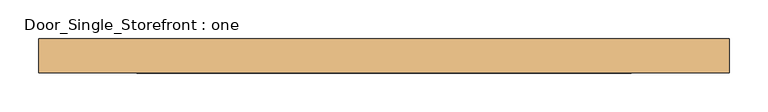
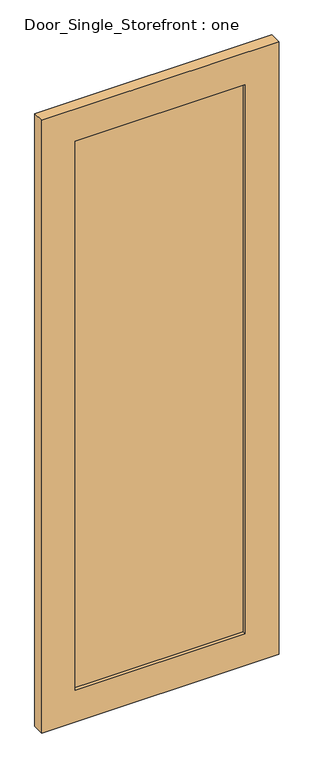
"""IFC4 building model written with IfcOpenShell, lengths in millimetres: door geometry, Door_Single_Storefront : one."""

from ifc_helpers import new_model, si_unit, frame, origin, place, context, project, spatial, polyline, outline, extrude, source, transform, mapped, element, save


def door_single_storefront_one_e372f670(model_context):
    return source(origin(), model_context, "Body", "SweptSolid", [
        extrude(outline(polyline([(319.88125, -6.35), (-319.88125, -6.35), (-319.88125, 12.7), (319.88125, 12.7), (319.88125, -6.35)])), frame((0.0, 0.0, 127.0), z_axis=(0.0, 0.0, 1.0), x_axis=(1.0, 0.0, 0.0)), (0.0, 0.0, 1.0), 2184.4),
        extrude(outline(polyline([(2438.4, -446.88125), (0.0, -446.88125), (0.0, 446.88125), (2438.4, 446.88125), (2438.4, -446.88125)]), holes=[polyline([(127.0, 319.88125), (127.0, -319.88125), (2311.4, -319.88125), (2311.4, 319.88125), (127.0, 319.88125)])]), frame((0.0, -19.05, 0.0), z_axis=(0.0, 1.0, 0.0), x_axis=(0.0, 0.0, 1.0)), (0.0, 0.0, 1.0), 44.45),
    ])


if __name__ == "__main__":
    model = new_model("IFC4")
    model_context = context("Model", 3, world=origin())
    ifc_project = project(units=[si_unit("LENGTHUNIT", "METRE", prefix="MILLI")], contexts=[model_context])
    site = spatial("IfcSite", under=ifc_project)
    building = spatial("IfcBuilding", under=site)
    placement = place(None, origin())
    door_single_storefront_one_shape = door_single_storefront_one_e372f670(model_context)
    element("IfcDoor", 1, ObjectType="Door_Single_Storefront : one", at=placement, inside=building, context=model_context, shape_type="MappedRepresentation", body=[
        mapped(door_single_storefront_one_shape, transform((0.0, 0.0, 0.0), x_axis=(1.0, 0.0, 0.0), y_axis=(0.0, 1.0, 0.0), z_axis=(0.0, 0.0, 1.0))),
    ])
    save(model, "model.ifc")

# Revit data of these elements
# Type "Door_Single_Storefront : one"
#   Type Mark = "27"
#   Analytic Construction = "<None>"
#   Stile_Width = 0' - 5"
#   Door_Thickness = 0' - 1 3/4"
#   Door_Offset = 0' - 1"
#   Glass_Material = SAFETY GLAZING
#   Frame_Material = INTERIOR GRADE ALUMINUM STOREFRONT W/ SAFETY GLAZING
#   Function = (empty or 0)
# Element 1 (IfcDoor, "Door_Single_Storefront : one")
#   Materials on its faces: "INTERIOR GRADE ALUMINUM STOREFRONT W/ SAFETY GLAZING", "SAFETY GLAZING"
# Materials
#   "SAFETY GLAZING": class "Glass", colour RGB 142 168 196, transparency 0.75, Description = "Soda Lime Glass", Cost = 0
#   "INTERIOR GRADE ALUMINUM STOREFRONT W/ SAFETY GLAZING": class "Metal", colour RGB 226 226 226, transparency 0, Description = "Aluminum 6061", Cost = 0
